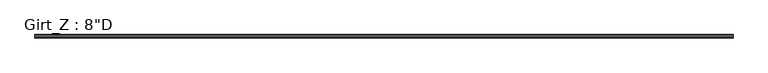
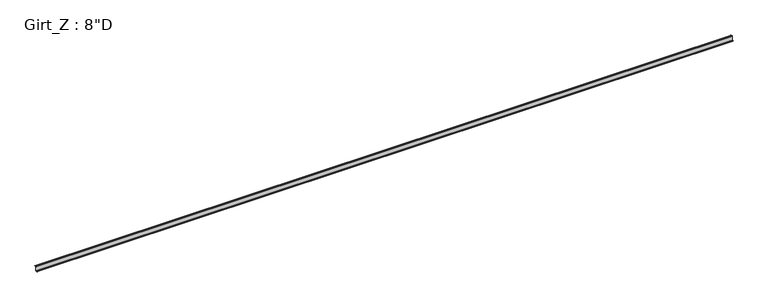
"""IFC4 building model written with IfcOpenShell, lengths in millimetres: beam geometry."""

from ifc_helpers import new_model, si_unit, point, frame, frame_2d, origin, place, context, project, spatial, polyline, circle_curve, trimmed, segment, composite_curve, outline, extrude, source, transform, mapped, element, save


def beam_0b2bf22b(model_context):
    return source(origin(), model_context, "Body", "SweptSolid", [
        extrude(outline(composite_curve([segment(polyline([(63.5, 101.6), (75.745104, 87.0068534), (73.6169367, 85.221109), (62.204539, 98.821875), (3.3005807, 98.821875)]), True, "CONTINUOUS"), segment(trimmed(circle_curve(frame_2d((3.3741066, 96.8381931)), 1.9850441), [point((3.3005807, 98.821875))], [point((1.3890625, 96.8381931))], True, "CARTESIAN"), True, "CONTINUOUS"), segment(polyline([(1.3890625, 96.8381931), (1.3890625, -96.8375)]), True, "CONTINUOUS"), segment(trimmed(circle_curve(frame_2d((-3.3734375, -96.8375)), 4.7625), [point((1.3890625, -96.8375))], [point((-3.3734375, -101.6))], False, "CARTESIAN"), True, "CONTINUOUS"), segment(polyline([(-3.3734375, -101.6), (-63.5, -101.6), (-75.745104, -87.0068534), (-73.6169367, -85.221109), (-62.204539, -98.821875), (-3.2694106, -98.821875)]), True, "CONTINUOUS"), segment(trimmed(circle_curve(frame_2d((-3.3748024, -96.8389339)), 1.9857399), [point((-3.2694106, -98.821875))], [point((-1.3890625, -96.8389339))], True, "CARTESIAN"), True, "CONTINUOUS"), segment(polyline([(-1.3890625, -96.8389339), (-1.3890625, 96.8375)]), True, "CONTINUOUS"), segment(trimmed(circle_curve(frame_2d((3.3734375, 96.8375)), 4.7625), [point((-1.3890625, 96.8375))], [point((3.3734375, 101.6))], False, "CARTESIAN"), True, "CONTINUOUS"), segment(polyline([(3.3734375, 101.6), (63.5, 101.6)]), True, "CONTINUOUS")], self_intersect=False)), frame((-15227.2999994, 0.0, 0.0), z_axis=(1.0, 0.0, 0.0), x_axis=(0.0, 1.0, 0.0)), (0.0, 0.0, 1.0), 30454.5999988),
    ])


if __name__ == "__main__":
    model = new_model("IFC4")
    model_context = context("Model", 3, world=origin())
    ifc_project = project(units=[si_unit("LENGTHUNIT", "METRE", prefix="MILLI")], contexts=[model_context])
    site = spatial("IfcSite", under=ifc_project)
    building = spatial("IfcBuilding", under=site)
    placement = place(None, origin())
    beam_shape = beam_0b2bf22b(model_context)
    element("IfcBeam", 1, ObjectType="Girt_Z : 8\"D", at=placement, inside=building, context=model_context, shape_type="MappedRepresentation", body=[
        mapped(beam_shape, transform((0.0, 0.0, 0.0), x_axis=(1.0, 0.0, 0.0), y_axis=(0.0, 1.0, 0.0), z_axis=(0.0, 0.0, 1.0))),
    ])
    save(model, "model.ifc")

# Revit data of these elements
# Type "Girt_Z : 8\"D"
#   Web_Thickness = 0' - 0 7/64"
#   Length [instance default] = 10' - 0"
#   Leg_1 = 0' - 2 1/2"
#   Height = 0' - 8"
#   Structural Material [instance default] = none
# Element 1 (IfcBeam, "Girt_Z : 8\"D")
#   Structural Material = Steel
#   Materials on its faces: "Steel"
# Materials
#   "Steel": class "Metal", colour RGB 118 118 114, transparency 0, Description = "Steel, mill finish", Cost = 0
